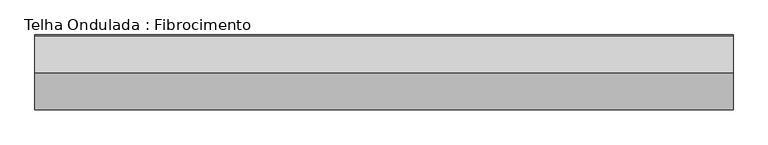
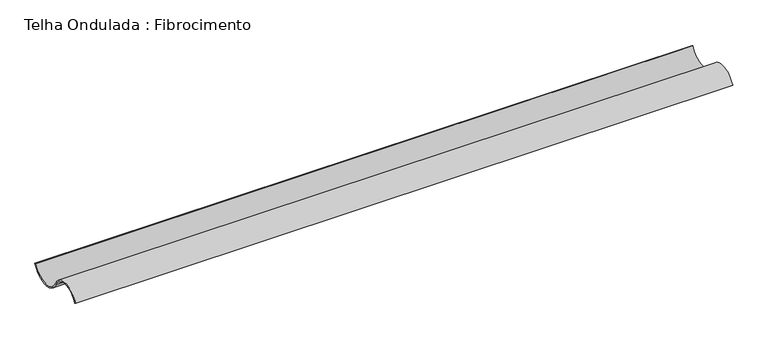
"""IFC4 building model written with IfcOpenShell, lengths in millimetres: beam geometry, Telha Ondulada : Fibrocimento."""

from ifc_helpers import new_model, si_unit, point, frame, frame_2d, origin, place, context, project, spatial, polyline, circle_curve, trimmed, segment, composite_curve, outline, extrude, source, transform, mapped, element, save


def telha_ondulada_fibrocimento_dedae922(model_context):
    return source(origin(), model_context, "Body", "SweptSolid", [
        extrude(outline(composite_curve([segment(trimmed(circle_curve(frame_2d((68.3970135, 71.7939461)), 66.7939461), [point((8.3970135, 42.4437972))], [point((128.3970135, 42.4437972))], True, "CARTESIAN"), True, "CONTINUOUS"), segment(polyline([(128.3970135, 42.4437972), (132.8884385, 40.2467307)]), True, "CONTINUOUS"), segment(trimmed(circle_curve(frame_2d((68.3970135, 71.7939461)), 71.7939461), [point((132.8884385, 40.2467307))], [point((3.9055884, 40.2467307))], False, "CARTESIAN"), True, "CONTINUOUS"), segment(trimmed(circle_curve(frame_2d((-51.6029865, 13.0936483)), 61.7939461), [point((3.9055884, 40.2467307))], [point((-107.1115615, 40.2467307))], True, "CARTESIAN"), True, "CONTINUOUS"), segment(polyline([(-107.1115615, 40.2467307), (-111.6029865, 42.4437972)]), True, "CONTINUOUS"), segment(trimmed(circle_curve(frame_2d((-51.6029865, 13.0936483)), 66.7939461), [point((-111.6029865, 42.4437972))], [point((8.3970135, 42.4437972))], False, "CARTESIAN"), True, "CONTINUOUS")], self_intersect=False)), frame((-1141.0240716, 0.0, 0.0), z_axis=(1.0, 0.0, 0.0), x_axis=(0.0, 1.0, 0.0)), (0.0, 0.0, 1.0), 2282.0481431),
    ])


if __name__ == "__main__":
    model = new_model("IFC4")
    model_context = context("Model", 3, world=origin())
    ifc_project = project(units=[si_unit("LENGTHUNIT", "METRE", prefix="MILLI")], contexts=[model_context])
    site = spatial("IfcSite", under=ifc_project)
    building = spatial("IfcBuilding", under=site)
    placement = place(None, origin())
    telha_ondulada_fibrocimento_shape = telha_ondulada_fibrocimento_dedae922(model_context)
    element("IfcBeam", 1, ObjectType="Telha Ondulada : Fibrocimento", at=placement, inside=building, context=model_context, shape_type="MappedRepresentation", body=[
        mapped(telha_ondulada_fibrocimento_shape, transform((0.0, 0.0, 0.0), x_axis=(1.0, 0.0, 0.0), y_axis=(0.0, 1.0, 0.0), z_axis=(0.0, 0.0, 1.0))),
    ])
    save(model, "model.ifc")

# Revit data of these elements
# Type "Telha Ondulada : Fibrocimento"
#   Description = "TELHA ONDULADA FIBROCIMENTO"
#   Cost = 5
#   Length [instance default] = 1.524 m
#   b = 0.07 m
#   h = 0.16 m
#   Structural Material = .TELHA DE FIBROCIMENTO
#   Assembly Code = ""
# Element 1 (IfcBeam, "Telha Ondulada : Fibrocimento")
#   Materials on its faces: ".TELHA DE FIBROCIMENTO"
# Materials
#   ".TELHA DE FIBROCIMENTO": class "CC_TELHADO", colour RGB 77 77 76, transparency 0, Description = "TELHA ONDULADA FIBROCIMENTO", Cost = 0
